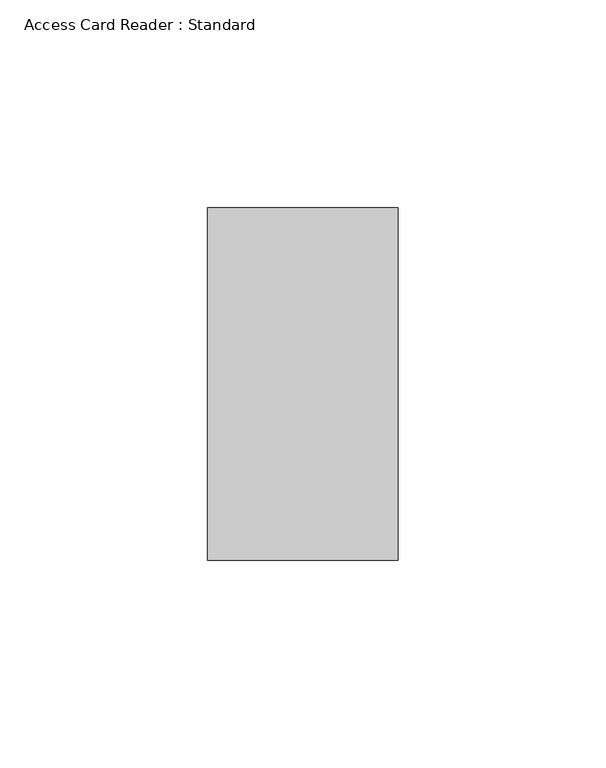
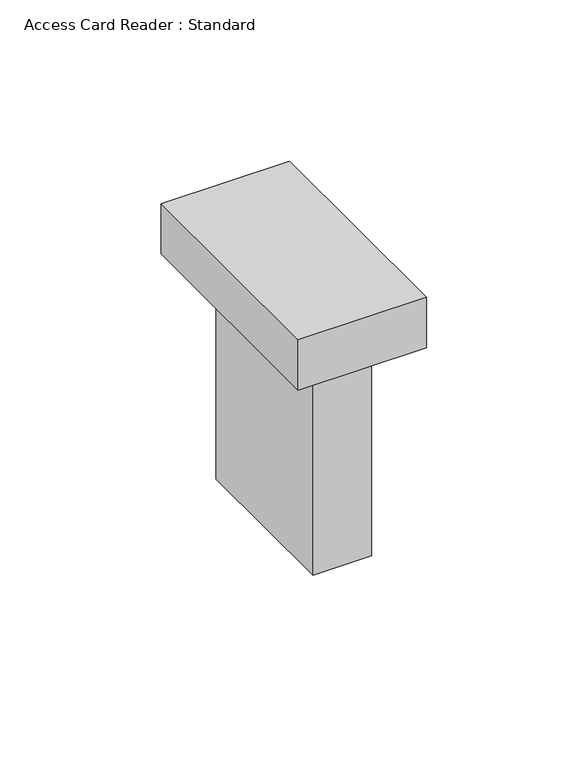
"""IFC4 building model written with IfcOpenShell, lengths in millimetres: proxy geometry, Access Card Reader : Standard."""

from ifc_helpers import new_model, si_unit, frame, origin, origin_with_axes, place, context, project, spatial, polyline, outline, extrude, source, transform, mapped, element, save


def access_card_reader_standard_2fd2a6f3(model_context):
    return source(origin(), model_context, "Body", "SweptSolid", [
        extrude(outline(polyline([(23.0, -85.0), (-23.0, -85.0), (-23.0, 0.0), (23.0, 0.0), (23.0, -85.0)])), origin_with_axes(), (0.0, 0.0, 1.0), 19.0),
        extrude(outline(polyline([(10.5, -72.5), (-10.5, -72.5), (-10.5, -12.5), (10.5, -12.5), (10.5, -72.5)])), frame((0.0, 0.0, -82.0), z_axis=(0.0, 0.0, 1.0), x_axis=(1.0, 0.0, 0.0)), (0.0, 0.0, 1.0), 82.0),
    ])


if __name__ == "__main__":
    model = new_model("IFC4")
    model_context = context("Model", 3, world=origin())
    ifc_project = project(units=[si_unit("LENGTHUNIT", "METRE", prefix="MILLI")], contexts=[model_context])
    site = spatial("IfcSite", under=ifc_project)
    building = spatial("IfcBuilding", under=site)
    placement = place(None, origin())
    access_card_reader_standard_shape = access_card_reader_standard_2fd2a6f3(model_context)
    element("IfcBuildingElementProxy", 1, Name="Access Card Reader : Standard", ObjectType="Access Card Reader : Standard", at=placement, inside=building, context=model_context, shape_type="MappedRepresentation", body=[
        mapped(access_card_reader_standard_shape, transform((0.0, 0.0, 0.0), x_axis=(1.0, 0.0, 0.0), y_axis=(0.0, 1.0, 0.0), z_axis=(0.0, 0.0, 1.0))),
    ])
    save(model, "model.ifc")

# Revit data of these elements
# Type "Access Card Reader : Standard"
#   Type Mark = "Access Card Reader"
#   Classification.OmniClass.21.Number = "21-04 70"
#   Classification.MasterFormat.Description = "Electronic Access Control and Intrusion Detection"
#   Classification.OmniClass.21.Description = "Electronic Safety and Security"
#   Classification.UniFormat.II.Description = "Access Control and Intrusion Detection"
#   Classification.MasterFormat.Number = "28 10 00"
#   Classification.OmniClass.23.Number = "23-29 13 00"
#   Classification.OmniClass.23.Description = "Security Access Controls"
#   Classification.UniFormat.II.Number = "D7010"
#   COBie.Type.CreatedBy = "info@mma.ie"
#   COBie.Type.CreatedOn = "2017-03-14T04:20:18"
#   COBie.Type.Name = "Access Card Reader"
#   COBie.Type.Category = "23-29 13 00 : Security Access Controls"
#   COBie.Type.Description = "Access Card Reader_Standard"
#   COBie.Type.AssetType = "Fixed"
#   COBie.Type.Manufacturer = ""
#   COBie.Type.ModelNumber = ""
#   COBie.Type.WarrantyDescription = ""
#   COBie.Type.ModelReference = ""
#   COBie.Type.Color = "Grey"
#   Units = "Volts"
#   Label = "CR"
#   Keynote = "28 13 43.A"
#   COBie.Type.ReplacementCost = 0
#   Default Elevation = 1200 mm
#   AC_Width = 46 mm
#   AC_Height = 85 mm
#   AC_Depth = 19 mm
#   COBie.Type = no
#   URL = ""
#   Model = ""
#   Manufacturer = ""
